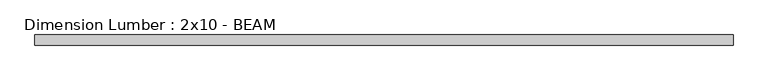
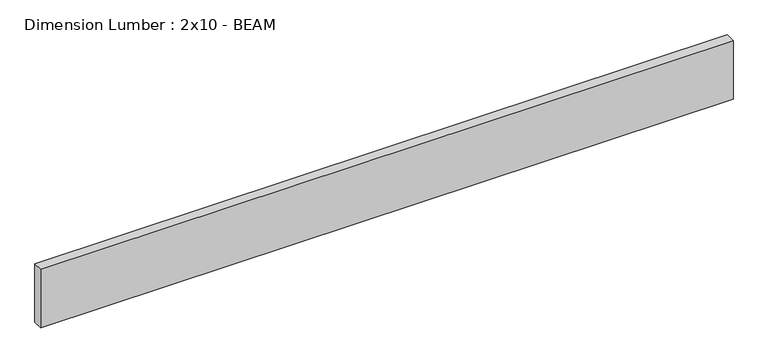
"""IFC4 building model written with IfcOpenShell, lengths in millimetres: beam geometry, Dimension Lumber : 2x10 - BEAM."""

from ifc_helpers import new_model, si_unit, frame, origin, place, context, project, spatial, polyline, outline, extrude, source, transform, mapped, element, save


def dimension_lumber_2x10_beam_8d0e8335(model_context):
    return source(origin(), model_context, "Body", "SweptSolid", [
        extrude(outline(polyline([(1314.45, 19.05), (1314.45, -19.05), (-1313.9963089, -19.05), (-1313.9963089, 19.05), (1314.45, 19.05)])), frame((0.0, 0.0, -117.475), z_axis=(0.0, 0.0, 1.0), x_axis=(1.0, 0.0, 0.0)), (0.0, 0.0, 1.0), 234.95),
    ])


if __name__ == "__main__":
    model = new_model("IFC4")
    model_context = context("Model", 3, world=origin())
    ifc_project = project(units=[si_unit("LENGTHUNIT", "METRE", prefix="MILLI")], contexts=[model_context])
    site = spatial("IfcSite", under=ifc_project)
    building = spatial("IfcBuilding", under=site)
    placement = place(None, origin())
    dimension_lumber_2x10_beam_shape = dimension_lumber_2x10_beam_8d0e8335(model_context)
    element("IfcBeam", 1, ObjectType="Dimension Lumber : 2x10 - BEAM", at=placement, inside=building, context=model_context, shape_type="MappedRepresentation", body=[
        mapped(dimension_lumber_2x10_beam_shape, transform((0.0, 0.0, 0.0), x_axis=(1.0, 0.0, 0.0), y_axis=(0.0, 1.0, 0.0), z_axis=(0.0, 0.0, 1.0))),
    ])
    save(model, "model.ifc")

# Revit data of these elements
# Type "Dimension Lumber : 2x10 - BEAM"
#   Assembly Code = "B10"
#   A = 0.0755556 SF
#   Length [instance default] = 5' - 0"
#   b = 0' - 1 1/2"
#   d = 0' - 9 1/4"
#   Structural Material = (3) SISTERED 2X10s AT BEAM
# Element 1 (IfcBeam, "Dimension Lumber : 2x10 - BEAM")
#   Materials on its faces: "(3) SISTERED 2X10s AT BEAM"
# Materials
#   "(3) SISTERED 2X10s AT BEAM": class "Wood", colour RGB 234 198 147, transparency 0, Description = "Pinus Echinata", Cost = 0
